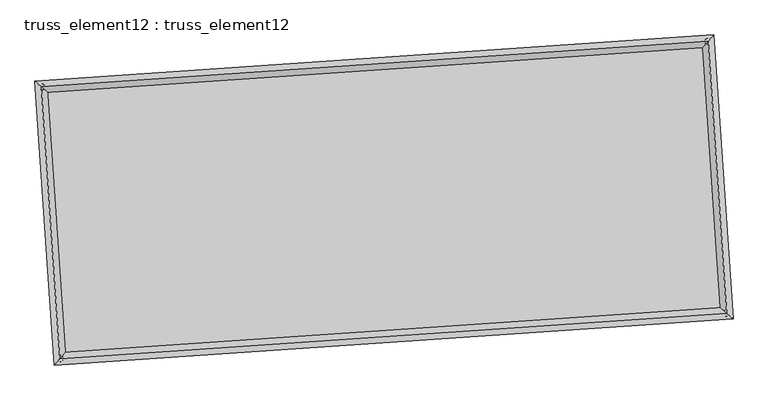
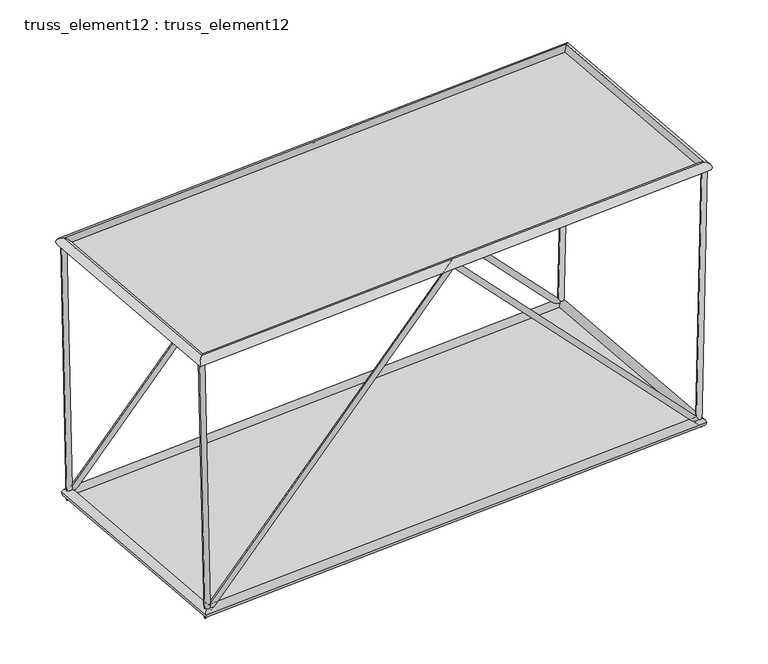
"""IFC4 building model written with IfcOpenShell, lengths in millimetres: plate geometry, truss_element12 : truss_element12."""

import ifcopenshell
import ifcopenshell.guid

model = None  # the IFC model being written
_history = None  # IfcOwnerHistory: only IFC2X3 demands one
_inside = {}  # id of a spatial element -> (the spatial element, [elements in it])
_under = {}  # id of a project, library or spatial element -> (it, [spatial elements below it])
_declared = {}  # id of a project -> (the project, [libraries it declares])
_typed = {}  # id of a type object -> (the type object, [elements of that type])
_made_of = {}  # id of a material, layer set ... -> (it, [elements and type objects made of it])


def new_model(schema):
    """Start an empty IFC model of exactly this schema.

    Asked for "IFC4X3", IfcOpenShell would pick the latest addendum, in which some entities
    have other attributes; the version numbers below select the first issue.
    IFC2X3 requires an IfcOwnerHistory on every rooted entity: one is made here for all.
    """
    global model, _history
    if schema == "IFC4X3":
        model = ifcopenshell.file(schema_version=(4, 3, 0, 0))
    else:
        model = ifcopenshell.file(schema=schema)
    _inside.clear()
    _under.clear()
    _declared.clear()
    _typed.clear()
    _made_of.clear()
    _history = None
    if model.schema == "IFC2X3":
        org = make("IfcOrganization", Name="unknown")
        user = make(
            "IfcPersonAndOrganization",
            ThePerson=make("IfcPerson", FamilyName="unknown"),
            TheOrganization=org,
        )
        app = make(
            "IfcApplication",
            ApplicationDeveloper=org,
            Version="unknown",
            ApplicationFullName="unknown",
            ApplicationIdentifier="unknown",
        )
        _history = make(
            "IfcOwnerHistory",
            OwningUser=user,
            OwningApplication=app,
            ChangeAction="ADDED",
            CreationDate=0,
        )
    return model


def make(cls, **values):
    """One entity of the class cls with the attributes given. An attribute that is None is left unset."""
    return model.create_entity(
        cls, **{name: value for name, value in values.items() if value is not None}
    )


def rooted(cls, **values):
    """An entity with a GlobalId (a new one), such as an element, a storey or a relation."""
    return make(cls, GlobalId=ifcopenshell.guid.new(), OwnerHistory=_history, **values)


def si_unit(unit_type, name, prefix=None):
    """IfcSIUnit, for example si_unit("LENGTHUNIT", "METRE", prefix="MILLI")."""
    return make("IfcSIUnit", UnitType=unit_type, Prefix=prefix, Name=name)


def assignment(units):
    """IfcUnitAssignment: the units of a project."""
    return None if units is None else make("IfcUnitAssignment", Units=units)


def point(xyz):
    """IfcCartesianPoint."""
    return None if xyz is None else make("IfcCartesianPoint", Coordinates=xyz)


def direction(xyz):
    """IfcDirection."""
    return None if xyz is None else make("IfcDirection", DirectionRatios=xyz)


def frame(location, z_axis=None, x_axis=None):
    """IfcAxis2Placement3D, a coordinate frame: its origin and axes. An axis left out is left unset."""
    return make(
        "IfcAxis2Placement3D",
        Location=point(location),
        Axis=direction(z_axis),
        RefDirection=direction(x_axis),
    )


def origin():
    """The frame at (0, 0, 0) with its axes left unset."""
    return frame((0.0, 0.0, 0.0))


def origin_with_axes():
    """The frame at (0, 0, 0) with the z axis (0, 0, 1) and the x axis (1, 0, 0) written out."""
    return frame((0.0, 0.0, 0.0), z_axis=(0.0, 0.0, 1.0), x_axis=(1.0, 0.0, 0.0))


def place(relative_to, where):
    """IfcLocalPlacement: puts the frame where relative to a parent placement (None: the world)."""
    return make(
        "IfcLocalPlacement", PlacementRelTo=relative_to, RelativePlacement=where
    )


def context(
    kind, dimensions, precision=None, world=None, true_north=None, identifier=None
):
    """IfcGeometricRepresentationContext, for example the 3D "Model" context."""
    return make(
        "IfcGeometricRepresentationContext",
        ContextIdentifier=identifier,
        ContextType=kind,
        CoordinateSpaceDimension=dimensions,
        Precision=precision,
        WorldCoordinateSystem=world,
        TrueNorth=true_north,
    )


def project(units=None, contexts=None):
    """IfcProject with its units and contexts."""
    return rooted(
        "IfcProject",
        Name="project",
        RepresentationContexts=contexts,
        UnitsInContext=assignment(units),
    )


def spatial(cls, under=None, at=None, **own):
    """A site, building, storey or space (cls), placed at a placement, below another one or the project."""
    s = rooted(cls, ObjectPlacement=at, **own)
    if under is not None:
        _under.setdefault(under.id(), (under, []))[1].append(s)
    return s


def polyline(points):
    """IfcPolyline through the points."""
    return make("IfcPolyline", Points=[point(p) for p in points])


def circle_curve(where, radius):
    """IfcCircle in the frame where."""
    return make("IfcCircle", Position=where, Radius=radius)


def ellipse_curve(where, semi_axis1, semi_axis2):
    """IfcEllipse in the frame where."""
    return make(
        "IfcEllipse", Position=where, SemiAxis1=semi_axis1, SemiAxis2=semi_axis2
    )


def outline(outer, holes=None, kind="AREA"):
    """IfcArbitraryClosedProfileDef: a profile drawn as a closed curve; with holes, ...WithVoids."""
    if holes is None:
        return make("IfcArbitraryClosedProfileDef", ProfileType=kind, OuterCurve=outer)
    return make(
        "IfcArbitraryProfileDefWithVoids",
        ProfileType=kind,
        OuterCurve=outer,
        InnerCurves=holes,
    )


def extrude(swept, where, along, depth):
    """IfcExtrudedAreaSolid: the profile swept, set in the frame where, extruded along a direction by depth."""
    return make(
        "IfcExtrudedAreaSolid",
        SweptArea=swept,
        Position=where,
        ExtrudedDirection=direction(along),
        Depth=depth,
    )


def shape(context_of_items, identifier, shape_type, items):
    """IfcShapeRepresentation: the items that make up one representation, for example the "Body"."""
    return make(
        "IfcShapeRepresentation",
        ContextOfItems=context_of_items,
        RepresentationIdentifier=identifier,
        RepresentationType=shape_type,
        Items=items,
    )


def source(mapping_origin, context_of_items, identifier, shape_type, items):
    """IfcRepresentationMap: a shape defined once, which mapped items show again and again."""
    return make(
        "IfcRepresentationMap",
        MappingOrigin=mapping_origin,
        MappedRepresentation=shape(context_of_items, identifier, shape_type, items),
    )


def transform(
    local_origin,
    x_axis=None,
    y_axis=None,
    z_axis=None,
    scale=None,
    scale2=None,
    scale3=None,
    uniform=True,
):
    """IfcCartesianTransformationOperator3D, or its non-uniform kind. x_axis, y_axis, z_axis: its Axis1, 2, 3."""
    if uniform:
        return make(
            "IfcCartesianTransformationOperator3D",
            Axis1=direction(x_axis),
            Axis2=direction(y_axis),
            LocalOrigin=point(local_origin),
            Scale=scale,
            Axis3=direction(z_axis),
        )
    return make(
        "IfcCartesianTransformationOperator3DnonUniform",
        Axis1=direction(x_axis),
        Axis2=direction(y_axis),
        LocalOrigin=point(local_origin),
        Scale=scale,
        Axis3=direction(z_axis),
        Scale2=scale2,
        Scale3=scale3,
    )


def mapped(mapping_source, mapping_target):
    """IfcMappedItem: shows the shape of a source again, moved by a transform."""
    return make(
        "IfcMappedItem", MappingSource=mapping_source, MappingTarget=mapping_target
    )


def made_of(thing, what):
    """Note that an element or type object is made of a material, layer set ...; save() writes the relation."""
    if what is not None:
        _made_of.setdefault(what.id(), (what, []))[1].append(thing)
    return thing


def element(
    cls,
    number,
    at=None,
    inside=None,
    cuts=None,
    type_object=None,
    material=None,
    context=None,
    identifier="Body",
    shape_type=None,
    held_by="IfcProductDefinitionShape",
    body=None,
    shapes=None,
    **own,
):
    """One element of the class cls, such as IfcWall. Its Tag is "e" and its number.

    at: its placement. inside: the storey or other place that contains it. cuts: it is an
    opening in that element (IfcRelVoidsElement). A single representation is given by context,
    identifier, shape_type and body (its items); several are given by shapes. held_by: the class
    of the entity that holds the representations. save() writes the other relations.
    """
    e = rooted(cls, Tag="e%d" % number, ObjectPlacement=at, **own)
    if body is not None:
        shapes = [shape(context, identifier, shape_type, body)]
    if shapes is not None:
        e.Representation = make(held_by, Representations=shapes)
    if inside is not None:
        _inside.setdefault(inside.id(), (inside, []))[1].append(e)
    if cuts is not None:
        rooted(
            "IfcRelVoidsElement", RelatingBuildingElement=cuts, RelatedOpeningElement=e
        )
    if type_object is not None:
        _typed.setdefault(type_object.id(), (type_object, []))[1].append(e)
    return made_of(e, material)


def aggregate(whole, parts):
    """IfcRelAggregates: a whole, such as a stair, and the parts it consists of."""
    return rooted("IfcRelAggregates", RelatingObject=whole, RelatedObjects=parts)


def save(model, path):
    """Write the relations noted so far, then the file.

    IfcRelAggregates (storeys below a building ...), IfcRelContainedInSpatialStructure (elements
    in a storey), IfcRelDefinesByType, IfcRelAssociatesMaterial and IfcRelDeclares: one each for
    every whole, place, type object, material and project.
    """
    for whole, parts in _under.values():
        aggregate(whole, parts)
    for where, things in _inside.values():
        rooted(
            "IfcRelContainedInSpatialStructure",
            RelatedElements=things,
            RelatingStructure=where,
        )
    for kind, things in _typed.values():
        rooted("IfcRelDefinesByType", RelatedObjects=things, RelatingType=kind)
    for what, things in _made_of.values():
        rooted("IfcRelAssociatesMaterial", RelatedObjects=things, RelatingMaterial=what)
    for by, libraries in _declared.values():
        rooted("IfcRelDeclares", RelatingContext=by, RelatedDefinitions=libraries)
    model.write(path)


def plane_surface(at):
    """IfcPlane: the flat surface through the origin of the frame at, square to its z axis."""
    return make("IfcPlane", Position=at)


def cylinder_surface(at, radius):
    """IfcCylindricalSurface: all points at the distance radius from the z axis of the frame at."""
    return make("IfcCylindricalSurface", Position=at, Radius=radius)


def advanced_brep(points, edges, surfaces, faces):
    """IfcAdvancedBrep: a solid bounded by faces that lie on surfaces and meet in shared edges.

    An edge is (start, end): straight between two places in points (the first is 0);
    or (start, end, curve); or (start, end, curve, False) where it runs against its curve.
    A face is (place in surfaces, loops), or (place, loops, False) where it looks against
    its surface's normal. A loop lists edges by number (the first is 1), with a minus sign
    where the edge is run from its end to its start. The first loop is the outer one.
    """
    corners = [point(p) for p in points]
    vertices = [make("IfcVertexPoint", VertexGeometry=c) for c in corners]
    made = []
    for start, end, *more in edges:
        made.append(
            make(
                "IfcEdgeCurve",
                EdgeStart=vertices[start],
                EdgeEnd=vertices[end],
                EdgeGeometry=more[0] if more else make("IfcPolyline", Points=[corners[start], corners[end]]),
                SameSense=more[1] if len(more) > 1 else True,
            )
        )
    hull = []
    for where, loops, *sense in faces:
        bounds = []
        for j, loop in enumerate(loops):
            ring = [make("IfcOrientedEdge", EdgeElement=made[abs(k) - 1], Orientation=k > 0) for k in loop]
            bounds.append(
                make(
                    "IfcFaceOuterBound" if j == 0 else "IfcFaceBound",
                    Bound=make("IfcEdgeLoop", EdgeList=ring),
                    Orientation=True,
                )
            )
        hull.append(make("IfcAdvancedFace", Bounds=bounds, FaceSurface=surfaces[where], SameSense=sense[0] if sense else True))
    return make("IfcAdvancedBrep", Outer=make("IfcClosedShell", CfsFaces=hull))


def truss_element12_truss_element12_301403ea(model_context):
    return source(origin(), model_context, "Body", "SolidModel", [
        advanced_brep(
        [(-3775.2469584, 2268.7026723, 4999.8808289), (-3874.3259881, 2255.3430826, 4997.6746502), (-3667.6082835, 2276.0421444, 121.4057073), (-3761.3785993, 2263.0445357, -121.4057073), (1063.2088881, 2598.6185838, 5070.903767), (1063.6647127, 2592.0458975, 4926.6740735), (5795.0228776, 2921.2629924, 121.4126479), (5889.7380994, 2921.1174961, -121.4126479), (5901.6721346, 2928.5349998, 4999.8930544), (6001.6480134, 2928.7482077, 4997.7071476)],
        [
            (0, 1, circle_curve(frame((-3824.7864732, 2262.0228775, 4998.7777396), z_axis=(-0.022058606365203313, -0.0015040925154301537, 0.9997555479170547), x_axis=(-0.1335964218064517, 0.9910347491932179, -0.0014566990247462872)), 50.0)),
            (1, 0, circle_curve(frame((-3824.7864732, 2262.0228775, 4998.7777396), z_axis=(-0.022058606365203313, -0.0015040925154301537, 0.9997555479170547), x_axis=(-0.1335964218064517, 0.9910347491932179, -0.0014566990247462872)), 50.0)),
            (0, 2),
            (2, 3, ellipse_curve(frame((-3714.4934414, 2269.54334, 0.0), z_axis=(-0.929831833890302, -0.06340169813126974, 0.3624817034806986), x_axis=(0.3616419769436298, 0.02465899167793033, 0.9319908876387853)), 130.5485583, 50.0)),
            (3, 1),
            (3, 2, ellipse_curve(frame((-3714.4934414, 2269.54334, 0.0), z_axis=(-0.929831833890302, -0.06340169813126974, 0.3624817034806986), x_axis=(0.3616419769436298, 0.02465899167793033, 0.9319908876387853)), 130.5485583, 50.0)),
            (2, 4),
            (4, 5, ellipse_curve(frame((1063.4368004, 2595.3322406, 4998.7889203), z_axis=(-0.9976833946750359, -0.06802823813325101, -5.297341116227876e-05), x_axis=(5.2850692750050104e-05, 3.603687834190323e-06, -0.9999999985969089)), 72.2718761, 50.0)),
            (5, 3),
            (5, 4, ellipse_curve(frame((1063.4368004, 2595.3322406, 4998.7889203), z_axis=(-0.9976833946750359, -0.06802823813325101, -5.297341116227876e-05), x_axis=(5.2850692750050104e-05, 3.603687834190323e-06, -0.9999999985969089)), 72.2718761, 50.0)),
            (4, 6),
            (6, 7, ellipse_curve(frame((5842.3804885, 2921.1902443, 0.0), z_axis=(-0.9297759208968333, -0.0633978856367901, -0.3626257644145411), x_axis=(-0.36178570414534755, -0.024668791889457083, 0.931934844816294)), 130.5638727, 50.0)),
            (7, 5),
            (7, 6, ellipse_curve(frame((5842.3804885, 2921.1902443, 0.0), z_axis=(-0.9297759208968333, -0.0633978856367901, -0.3626257644145411), x_axis=(-0.36178570414534755, -0.024668791889457083, 0.931934844816294)), 130.5638727, 50.0)),
            (8, 9, circle_curve(frame((5951.660074, 2928.6416038, 4998.800101), z_axis=(0.021855917096442128, 0.0014902719046874222, 0.9997600201936081), x_axis=(-0.0021641430734946694, 0.9999966166591524, -0.001443313897180082)), 50.0)),
            (9, 8, circle_curve(frame((5951.660074, 2928.6416038, 4998.800101), z_axis=(0.021855917096442128, 0.0014902719046874222, 0.9997600201936081), x_axis=(-0.0021641430734946694, 0.9999966166591524, -0.001443313897180082)), 50.0)),
            (6, 8),
            (9, 7),
        ],
        [
            plane_surface(frame((-3824.7864732, 2312.0228209, 4998.8529625), z_axis=(-0.022058606365203737, -0.0015040925154315642, 0.9997555479170548), x_axis=(0.9997566793401409, -3.318625963721899e-05, 0.022058581401513063))),
            cylinder_surface(frame((-3824.7864732, 2262.0228775, 4998.7777396), z_axis=(-0.022058606365203317, -0.0015040925154301541, 0.9997555479170549), x_axis=(-0.1335964218064517, 0.9910347491932179, -0.0014566990247462872)), 50.0),
            cylinder_surface(frame((-3714.4934414, 2269.54334, 0.0), z_axis=(-0.690191184581497, -0.04706151321429389, -0.7220951064091011), x_axis=(-0.020415630046097626, 0.998752117142888, -0.04557861946592952)), 50.0),
            cylinder_surface(frame((1063.4368004, 2595.3322406, 4998.7889203), z_axis=(-0.6902675071609956, -0.04706671736086042, 0.7220218090020676), x_axis=(-0.11534041081619323, 0.9922795571850488, -0.04558365963144496)), 50.0),
            plane_surface(frame((5951.660074, 2878.6416593, 4998.8746324), z_axis=(0.021855917096441312, 0.0014902719046848058, 0.9997600201936081), x_axis=(0.9997611309147169, -3.257904132603074e-05, -0.02185589281481271))),
            cylinder_surface(frame((5842.3804885, 2921.1902443, 0.0), z_axis=(-0.021855917096442128, -0.0014902719046874222, -0.9997600201936081), x_axis=(-0.0021641430734946694, 0.9999966166591524, -0.001443313897180082)), 50.0),
        ],
        [
            (0, [[1, 2]]),
            (1, [[-1, 3, 4, 5]]),
            (1, [[-2, -5, 6, -3]]),
            (2, [[-4, 7, 8, 9]]),
            (2, [[-6, -9, 10, -7]]),
            (3, [[-8, 11, 12, 13]]),
            (3, [[-10, -13, 14, -11]]),
            (4, [[15, 16]]),
            (5, [[-12, 17, -16, 18]]),
            (5, [[-14, -18, -15, -17]]),
        ],
    ),
        advanced_brep(
        [(-3503.1340054, -1722.030912, 4999.8808289), (-3602.2130352, -1735.3905017, 4997.6746502), (-3395.4953306, -1714.6914399, 121.4057073), (-3489.2656464, -1727.6890486, -121.4057073), (1335.321841, -1392.1150005, 5070.903767), (1335.7776656, -1398.6876868, 4926.6740735), (6067.1358305, -1069.4705919, 121.4126479), (6161.8510524, -1069.6160882, -121.4126479), (6173.7850875, -1062.1985845, 4999.8930544), (6273.7609663, -1061.9853766, 4997.7071476)],
        [
            (0, 1, circle_curve(frame((-3552.6735203, -1728.7107068, 4998.7777396), z_axis=(-0.0220586063652034, -0.0015040925154302146, 0.9997555479170548), x_axis=(-0.13359642180645137, 0.9910347491932178, -0.001456699024746231)), 50.0)),
            (1, 0, circle_curve(frame((-3552.6735203, -1728.7107068, 4998.7777396), z_axis=(-0.0220586063652034, -0.0015040925154302146, 0.9997555479170548), x_axis=(-0.13359642180645137, 0.9910347491932178, -0.001456699024746231)), 50.0)),
            (0, 2),
            (2, 3, ellipse_curve(frame((-3442.3804885, -1721.1902443, 0.0), z_axis=(-0.929831833890302, -0.06340169813126961, 0.3624817034806985), x_axis=(0.3616419769436297, 0.024658991677930217, 0.9319908876387852)), 130.5485583, 50.0)),
            (3, 1),
            (3, 2, ellipse_curve(frame((-3442.3804885, -1721.1902443, 0.0), z_axis=(-0.929831833890302, -0.06340169813126961, 0.3624817034806985), x_axis=(0.3616419769436297, 0.024658991677930217, 0.9319908876387852)), 130.5485583, 50.0)),
            (2, 4),
            (4, 5, ellipse_curve(frame((1335.5497533, -1395.4013437, 4998.7889203), z_axis=(-0.9976833946750359, -0.06802823813325097, -5.297341116235902e-05), x_axis=(5.285069275020386e-05, 3.6036878343633e-06, -0.9999999985969089)), 72.2718761, 50.0)),
            (5, 3),
            (5, 4, ellipse_curve(frame((1335.5497533, -1395.4013437, 4998.7889203), z_axis=(-0.9976833946750359, -0.06802823813325097, -5.297341116235902e-05), x_axis=(5.285069275020386e-05, 3.6036878343633e-06, -0.9999999985969089)), 72.2718761, 50.0)),
            (4, 6),
            (6, 7, ellipse_curve(frame((6114.4934414, -1069.54334, 0.0), z_axis=(-0.9297759208968333, -0.06339788563679019, -0.3626257644145409), x_axis=(-0.36178570414534744, -0.024668791889457125, 0.9319348448162941)), 130.5638727, 50.0)),
            (7, 5),
            (7, 6, ellipse_curve(frame((6114.4934414, -1069.54334, 0.0), z_axis=(-0.9297759208968333, -0.06339788563679019, -0.3626257644145409), x_axis=(-0.36178570414534744, -0.024668791889457125, 0.9319348448162941)), 130.5638727, 50.0)),
            (8, 9, circle_curve(frame((6223.7730269, -1062.0919805, 4998.800101), z_axis=(0.021855917096442214, 0.0014902719046874218, 0.9997600201936081), x_axis=(-0.002164143073494981, 0.9999966166591524, -0.0014433138971800747)), 50.0)),
            (9, 8, circle_curve(frame((6223.7730269, -1062.0919805, 4998.800101), z_axis=(0.021855917096442214, 0.0014902719046874218, 0.9997600201936081), x_axis=(-0.002164143073494981, 0.9999966166591524, -0.0014433138971800747)), 50.0)),
            (6, 8),
            (9, 7),
        ],
        [
            plane_surface(frame((-3552.6735203, -1678.7107634, 4998.8529625), z_axis=(-0.022058606365203737, -0.0015040925154315764, 0.9997555479170548), x_axis=(0.9997566793401409, -3.318625963721899e-05, 0.022058581401513063))),
            cylinder_surface(frame((-3552.6735203, -1728.7107068, 4998.7777396), z_axis=(-0.022058606365203397, -0.0015040925154302142, 0.9997555479170546), x_axis=(-0.13359642180645137, 0.9910347491932178, -0.001456699024746231)), 50.0),
            cylinder_surface(frame((-3442.3804885, -1721.1902443, 0.0), z_axis=(-0.6901911845814968, -0.04706151321429372, -0.7220951064091014), x_axis=(-0.02041563004609754, 0.998752117142888, -0.04557861946592936)), 50.0),
            cylinder_surface(frame((1335.5497533, -1395.4013437, 4998.7889203), z_axis=(-0.6902675071609955, -0.04706671736086049, 0.7220218090020676), x_axis=(-0.11534041081619317, 0.9922795571850488, -0.04558365963144479)), 50.0),
            plane_surface(frame((6223.7730269, -1112.091925, 4998.8746324), z_axis=(0.02185591709644131, 0.001490271904684816, 0.9997600201936081), x_axis=(0.9997611309147169, -3.257904132558665e-05, -0.02185589281481271))),
            cylinder_surface(frame((6114.4934414, -1069.54334, 0.0), z_axis=(-0.021855917096442214, -0.0014902719046874218, -0.9997600201936081), x_axis=(-0.002164143073494981, 0.9999966166591524, -0.0014433138971800747)), 50.0),
        ],
        [
            (0, [[1, 2]]),
            (1, [[-1, 3, 4, 5]]),
            (1, [[-2, -5, 6, -3]]),
            (2, [[-4, 7, 8, 9]]),
            (2, [[-6, -9, 10, -7]]),
            (3, [[-8, 11, 12, 13]]),
            (3, [[-10, -13, 14, -11]]),
            (4, [[15, 16]]),
            (5, [[-12, 17, -16, 18]]),
            (5, [[-14, -18, -15, -17]]),
        ],
    ),
        advanced_brep(
        [(-3552.6677087, -1728.7042655, 4908.7777398), (-3552.679332, -1728.7171481, 5088.7777394), (-3824.7931055, 2262.0284703, 5088.7777394), (-3824.779841, 2262.0172847, 4908.7777398), (5951.6654758, 2928.6480171, 5088.8001008), (5951.6546721, 2928.6351904, 4908.8001012), (6223.7792493, -1062.0976013, 5088.8001008), (6223.7668045, -1062.0863598, 4908.8001012)],
        [
            (0, 1, ellipse_curve(frame((-3552.6735203, -1728.7107068, 4998.7777396), z_axis=(-0.7535719234036206, 0.6573654662782067, -1.6135980941074279e-06), x_axis=(-0.6573654662762446, -0.7535719234053321, -1.6135980941074448e-06)), 127.2792206, 90.0)),
            (1, 2),
            (2, 3, ellipse_curve(frame((-3824.7864732, 2262.0228775, 4998.7777396), z_axis=(-0.6573654662762446, -0.7535719234053322, -1.6135980941074584e-06), x_axis=(0.7535719234036207, -0.6573654662782067, 1.6135980941074419e-06)), 127.2792206, 90.0)),
            (3, 0),
            (1, 0, ellipse_curve(frame((-3552.6735203, -1728.7107068, 4998.7777396), z_axis=(-0.7535719234036206, 0.6573654662782067, -1.6135980941074279e-06), x_axis=(-0.6573654662762446, -0.7535719234053321, -1.6135980941074448e-06)), 127.2792206, 90.0)),
            (3, 2, ellipse_curve(frame((-3824.7864732, 2262.0228775, 4998.7777396), z_axis=(-0.6573654662762446, -0.7535719234053322, -1.6135980941074584e-06), x_axis=(0.7535719234036207, -0.6573654662782067, 1.6135980941074419e-06)), 127.2792206, 90.0)),
            (2, 4),
            (4, 5, ellipse_curve(frame((5951.660074, 2928.6416038, 4998.800101), z_axis=(-0.7535719234036206, 0.6573654662782067, -1.6135980941074558e-06), x_axis=(-0.6573654662762446, -0.753571923405332, -1.6135980941074438e-06)), 127.2792206, 90.0)),
            (5, 3),
            (5, 4, ellipse_curve(frame((5951.660074, 2928.6416038, 4998.800101), z_axis=(-0.7535719234036206, 0.6573654662782067, -1.6135980941074558e-06), x_axis=(-0.6573654662762446, -0.753571923405332, -1.6135980941074438e-06)), 127.2792206, 90.0)),
            (4, 6),
            (6, 7, ellipse_curve(frame((6223.7730269, -1062.0919805, 4998.800101), z_axis=(0.6573654662762446, 0.7535719234053322, 1.6135980941074302e-06), x_axis=(-0.7535719234036207, 0.6573654662782067, -1.6135980941074425e-06)), 127.2792206, 90.0)),
            (7, 5),
            (7, 6, ellipse_curve(frame((6223.7730269, -1062.0919805, 4998.800101), z_axis=(0.6573654662762446, 0.7535719234053322, 1.6135980941074302e-06), x_axis=(-0.7535719234036207, 0.6573654662782067, -1.6135980941074425e-06)), 127.2792206, 90.0)),
            (6, 1),
            (0, 7),
        ],
        [
            cylinder_surface(frame((-3552.6735203, -1728.7107068, 4998.7777396), z_axis=(0.06802823822870047, -0.9976833960748768, 0.0), x_axis=(-0.9976833936796621, -0.06802823806537987, -6.929323564644417e-05)), 90.0),
            cylinder_surface(frame((-3824.7864732, 2262.0228775, 4998.7777396), z_axis=(-0.9976833960722788, -0.06802823822852337, -2.2819723089061332e-06), x_axis=(-0.06802823792339617, 0.997683393845226, -6.701126334266164e-05)), 90.0),
            cylinder_surface(frame((5951.660074, 2928.6416038, 4998.800101), z_axis=(-0.0680282382287004, 0.9976833960748768, 0.0), x_axis=(0.9976833939847893, 0.06802823808618527, -6.472929103887912e-05)), 90.0),
            cylinder_surface(frame((6223.7730269, -1062.0919805, 4998.800101), z_axis=(0.997683396072279, 0.06802823822852329, 2.281972308906114e-06), x_axis=(0.06802823822852329, -0.9976833938244205, -6.701126334266163e-05)), 90.0),
        ],
        [
            (0, [[1, 2, 3, 4]]),
            (0, [[5, -4, 6, -2]]),
            (1, [[-3, 7, 8, 9]]),
            (1, [[-6, -9, 10, -7]]),
            (2, [[-8, 11, 12, 13]]),
            (2, [[-10, -13, 14, -11]]),
            (3, [[-12, 15, -1, 16]]),
            (3, [[-14, -16, -5, -15]]),
        ],
    ),
        advanced_brep(
        [(-3358.7115243, -1625.2761972, 0.0), (-3526.0494527, -1817.1042913, 0.0), (-3810.4074885, 2353.2123043, 0.0), (-3618.5793943, 2185.8743758, 0.0), (5926.0494527, 3017.1042913, 0.0), (5758.7115243, 2825.2761972, 0.0), (6210.4074885, -1153.2123043, 0.0), (6018.5793943, -985.8743758, 0.0)],
        [
            (0, 1, ellipse_curve(frame((-3442.3804885, -1721.1902443, 0.0), z_axis=(-0.7535719234054578, 0.6573654662780809, 0.0), x_axis=(-0.6573654662780808, -0.7535719234054579, 0.0)), 127.2792206, 90.0)),
            (1, 2),
            (2, 3, ellipse_curve(frame((-3714.4934414, 2269.54334, 0.0), z_axis=(-0.6573654662780809, -0.753571923405458, 0.0), x_axis=(0.7535719234054579, -0.6573654662780808, 0.0)), 127.2792206, 90.0)),
            (3, 0),
            (1, 0, ellipse_curve(frame((-3442.3804885, -1721.1902443, 0.0), z_axis=(-0.7535719234054578, 0.6573654662780809, 0.0), x_axis=(-0.6573654662780808, -0.7535719234054579, 0.0)), 127.2792206, 90.0)),
            (3, 2, ellipse_curve(frame((-3714.4934414, 2269.54334, 0.0), z_axis=(-0.6573654662780809, -0.753571923405458, 0.0), x_axis=(0.7535719234054579, -0.6573654662780808, 0.0)), 127.2792206, 90.0)),
            (2, 4),
            (4, 5, ellipse_curve(frame((5842.3804885, 2921.1902443, 0.0), z_axis=(-0.7535719234054578, 0.657365466278081, 0.0), x_axis=(-0.6573654662780812, -0.7535719234054576, 0.0)), 127.2792206, 90.0)),
            (5, 3),
            (5, 4, ellipse_curve(frame((5842.3804885, 2921.1902443, 0.0), z_axis=(-0.7535719234054578, 0.657365466278081, 0.0), x_axis=(-0.6573654662780812, -0.7535719234054576, 0.0)), 127.2792206, 90.0)),
            (4, 6),
            (6, 7, ellipse_curve(frame((6114.4934414, -1069.54334, 0.0), z_axis=(0.657365466278081, 0.7535719234054576, 0.0), x_axis=(-0.7535719234054575, 0.6573654662780813, 0.0)), 127.2792206, 90.0)),
            (7, 5),
            (7, 6, ellipse_curve(frame((6114.4934414, -1069.54334, 0.0), z_axis=(0.657365466278081, 0.7535719234054576, 0.0), x_axis=(-0.7535719234054575, 0.6573654662780813, 0.0)), 127.2792206, 90.0)),
            (6, 1),
            (0, 7),
        ],
        [
            cylinder_surface(frame((-3442.3804885, -1721.1902443, 0.0), z_axis=(0.0680282382287013, -0.9976833960748767, 0.0), x_axis=(-0.9976833960748767, -0.0680282382287013, 0.0)), 90.0),
            cylinder_surface(frame((-3714.4934414, 2269.54334, 0.0), z_axis=(-0.9976833960748767, -0.06802823822870113, 0.0), x_axis=(-0.06802823822870113, 0.9976833960748767, 0.0)), 90.0),
            cylinder_surface(frame((5842.3804885, 2921.1902443, 0.0), z_axis=(-0.06802823822870095, 0.9976833960748767, 0.0), x_axis=(0.9976833960748767, 0.06802823822870095, 0.0)), 90.0),
            cylinder_surface(frame((6114.4934414, -1069.54334, 0.0), z_axis=(0.9976833960748767, 0.06802823822870079, 0.0), x_axis=(0.06802823822870079, -0.9976833960748767, 0.0)), 90.0),
        ],
        [
            (0, [[1, 2, 3, 4]]),
            (0, [[5, -4, 6, -2]]),
            (1, [[-3, 7, 8, 9]]),
            (1, [[-6, -9, 10, -7]]),
            (2, [[-8, 11, 12, 13]]),
            (2, [[-10, -13, 14, -11]]),
            (3, [[-12, 15, -1, 16]]),
            (3, [[-14, -16, -5, -15]]),
        ],
    ),
        extrude(outline(polyline([(-3442.3804885, -1721.1902443), (-3714.4934414, 2269.54334), (5842.3804885, 2921.1902443), (6114.4934414, -1069.54334), (-3442.3804885, -1721.1902443)])), origin_with_axes(), (0.0, 0.0, 1.0), 20.0),
        extrude(outline(polyline([(-2000.0, 4899.5736451), (2000.0, 4899.5736451), (2000.0, -4899.5736452), (-2000.0, -4899.5736452), (-2000.0, 4899.5736451)])), frame((1199.4932768, 599.9654485, 4998.7889203), z_axis=(-2.276685882898288e-06, -1.5523855586156375e-07, 0.9999999999973964), x_axis=(-0.06802823822870063, 0.9976833960748767, 0.0)), (0.0, 0.0, 1.0), 20.0),
    ])


if __name__ == "__main__":
    model = new_model("IFC4")
    model_context = context("Model", 3, world=origin())
    ifc_project = project(units=[si_unit("LENGTHUNIT", "METRE", prefix="MILLI")], contexts=[model_context])
    site = spatial("IfcSite", under=ifc_project)
    building = spatial("IfcBuilding", under=site)
    placement = place(None, origin())
    truss_element12_truss_element12_shape = truss_element12_truss_element12_301403ea(model_context)
    element("IfcPlate", 1, ObjectType="truss_element12 : truss_element12", at=placement, inside=building, context=model_context, shape_type="MappedRepresentation", body=[
        mapped(truss_element12_truss_element12_shape, transform((0.0, 0.0, 0.0), x_axis=(1.0, 0.0, 0.0), y_axis=(0.0, 1.0, 0.0), z_axis=(0.0, 0.0, 1.0))),
    ])
    save(model, "model.ifc")

# Revit data of these elements
# Type "truss_element12 : truss_element12"
#   steellbar1 = 90 mm
#   steelbar2 = 50 mm
#   offset1 = 5000 mm
#   M = Default Roof
# Element 1 (IfcPlate, "truss_element12 : truss_element12")
#   Materials on its faces: "Default Roof"
# Materials
#   "Default Roof": class "Miscellaneous", colour RGB 0 127 0, transparency 0, Comments = "Rendering appearance not upgraded Rendering appearance not upgraded ", Cost = 0
